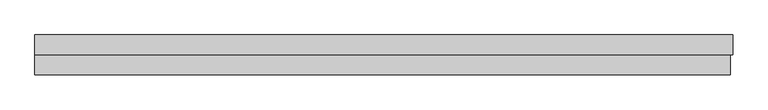
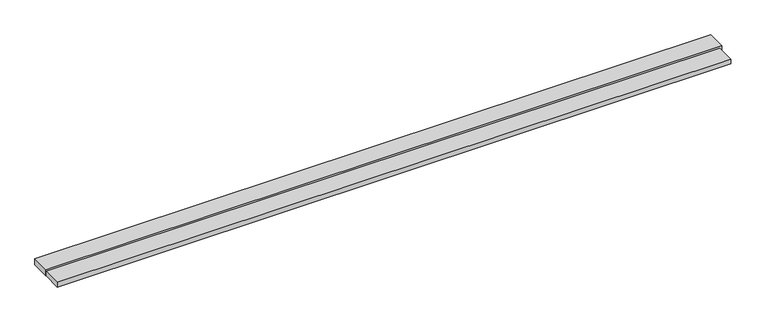
"""IFC4 building model written with IfcOpenShell, lengths in millimetres: proxy geometry, Generic Models 3:Generic Models 1:6:Generic Models 1:6 : Generic Models 3:Generic Models 1:300625:350611:Generic Models 1:6:Generic Models 1:6 : Generic Models 3:Generic Models 1:300625:350611 : Generic Models 3:Generic Models 1:6:Generic Models 1:6 : Generic Models 3:Generic Models 1:300625:350611:7 : Generic Models 3:Generic Models 1:6:Generic Models 1:6 : Generic Models 3:Generic Models 1:300625:350611:Generic Models 1:6:Generic Models 1:6 : Generic Models 3:Generic Models 1:300625:350611 : Generic Models 3:Generic Models 1:6:Generic Models 1:6 : Generic Models 3:Generic Models 1:300625:350611:301824."""

from ifc_helpers import new_model, si_unit, frame, origin, place, context, project, spatial, polyline, outline, extrude, source, transform, mapped, element, save


def generic_models_6d8d0986(model_context):
    return source(origin(), model_context, "Body", "SweptSolid", [
        extrude(outline(polyline([(596176.4867239, -579070.6520914), (596176.4867239, -579140.3913841), (593738.0867239, -579140.3913841), (593738.0867239, -579070.6520914), (596176.4867239, -579070.6520914)])), frame((0.0, 0.0, 1.3647904), z_axis=(0.0, 0.0, 1.0), x_axis=(1.0, 0.0, 0.0)), (0.0, 0.0, 1.0), 17.6585659),
        extrude(outline(polyline([(596184.8210989, -579000.6913841), (596184.8210989, -579070.1283008), (593738.0867239, -579070.1283008), (593738.0867239, -579000.6913841), (596184.8210989, -579000.6913841)])), frame((0.0, 0.0, 1.3647904), z_axis=(0.0, 0.0, 1.0), x_axis=(1.0, 0.0, 0.0)), (0.0, 0.0, 1.0), 23.478574),
    ])


if __name__ == "__main__":
    model = new_model("IFC4")
    model_context = context("Model", 3, world=origin())
    ifc_project = project(units=[si_unit("LENGTHUNIT", "METRE", prefix="MILLI")], contexts=[model_context])
    site = spatial("IfcSite", under=ifc_project)
    building = spatial("IfcBuilding", under=site)
    placement = place(None, origin())
    generic_models_shape = generic_models_6d8d0986(model_context)
    element("IfcBuildingElementProxy", 1, Name="Generic Models 3:Generic Models 1:6:Generic Models 1:6 : Generic Models 3:Generic Models 1:300625:350611:Generic Models 1:6:Generic Models 1:6 : Generic Models 3:Generic Models 1:300625:350611 : Generic Models 3:Generic Models 1:6:Generic Models 1:6 : Generic Models 3:Generic Models 1:300625:350611:7 : Generic Models 3:Generic Models 1:6:Generic Models 1:6 : Generic Models 3:Generic Models 1:300625:350611:Generic Models 1:6:Generic Models 1:6 : Generic Models 3:Generic Models 1:300625:350611 : Generic Models 3:Generic Models 1:6:Generic Models 1:6 : Generic Models 3:Generic Models 1:300625:350611:301824", ObjectType="Generic Models 3:Generic Models 1:6:Generic Models 1:6 : Generic Models 3:Generic Models 1:300625:350611:Generic Models 1:6:Generic Models 1:6 : Generic Models 3:Generic Models 1:300625:350611 : Generic Models 3:Generic Models 1:6:Generic Models 1:6 : Generic Models 3:Generic Models 1:300625:350611:7 : Generic Models 3:Generic Models 1:6:Generic Models 1:6 : Generic Models 3:Generic Models 1:300625:350611:Generic Models 1:6:Generic Models 1:6 : Generic Models 3:Generic Models 1:300625:350611 : Generic Models 3:Generic Models 1:6:Generic Models 1:6 : Generic Models 3:Generic Models 1:300625:350611:301824", at=placement, inside=building, context=model_context, shape_type="MappedRepresentation", body=[
        mapped(generic_models_shape, transform((0.0, 0.0, 0.0), x_axis=(1.0, 0.0, 0.0), y_axis=(0.0, 1.0, 0.0), z_axis=(0.0, 0.0, 1.0))),
    ])
    save(model, "model.ifc")

# Revit data of these elements
# Type "Generic Models 3:Generic Models 1:6:Generic Models 1:6 : Generic Models 3:Generic Models 1:300625:350611:Generic Models 1:6:Generic Models 1:6 : Generic Models 3:Generic Models 1:300625:350611 : Generic Models 3:Generic Models 1:6:Generic Models 1:6 : Generic Models 3:Generic Models 1:300625:350611:7 : Generic Models 3:Generic Models 1:6:Generic Models 1:6 : Generic Models 3:Generic Models 1:300625:350611:Generic Models 1:6:Generic Models 1:6 : Generic Models 3:Generic Models 1:300625:350611 : Generic Models 3:Generic Models 1:6:Generic Models 1:6 : Generic Models 3:Generic Models 1:300625:350611:301824"
#   NameOverride = "Generic Models 3:Generic Models 1:6:Generic Models 1:6 : Generic Models 3:Generic Models 1:300625:350611:Generic Models 1:6:Generic Models 1:6 : Generic Models 3:Generic Models 1:300625:350611 : Generic Models 3:Generic Models 1:6:Generic Models 1:6 : Generic Models 3:Generic Models 1:300625:350611:301824"
#   ObjectTypeOverride = "Generic Models 1:6:Generic Models 1:6 : Generic Models 3:Generic Models 1:300625:350611 : Generic Models 3:Generic Models 1:6:Generic Models 1:6 : Generic Models 3:Generic Models 1:300625:350611"
#   Reference = "Generic Models 1"
#   Tag = "301824"
# Element 1 (IfcBuildingElementProxy, "Generic Models 3:Generic Models 1:6:Generic Models 1:6 : Generic Models 3:Generic Models 1:300625:350611:Generic Models 1:6:Generic Models 1:6 : Generic Models 3:Generic Models 1:300625:350611 : Generic Models 3:Generic Models 1:6:Generic Models 1:6 : Generic Models 3:Generic Models 1:300625:350611:7 : Generic Models 3:Generic Models 1:6:Generic Models 1:6 : Generic Models 3:Generic Models 1:300625:350611:Generic Models 1:6:Generic Models 1:6 : Generic Models 3:Generic Models 1:300625:350611 : Generic Models 3:Generic Models 1:6:Generic Models 1:6 : Generic Models 3:Generic Models 1:300625:350611:301824")
#   Materials on its faces: "EXTRUDED POLYSTYRENE (XPS) RIGID FOAM INSULATION (FOAMULAR® 250 OR SIMILAR)"
# Materials
#   "EXTRUDED POLYSTYRENE (XPS) RIGID FOAM INSULATION (FOAMULAR® 250 OR SIMILAR)": class "Unassigned", colour RGB 247 185 194, transparency 0, Cost = 0
